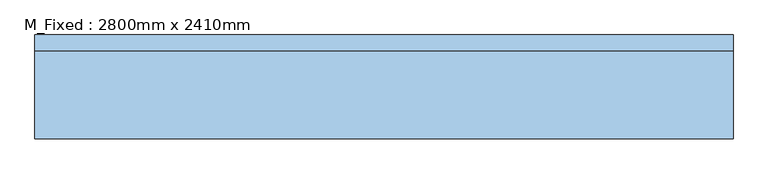
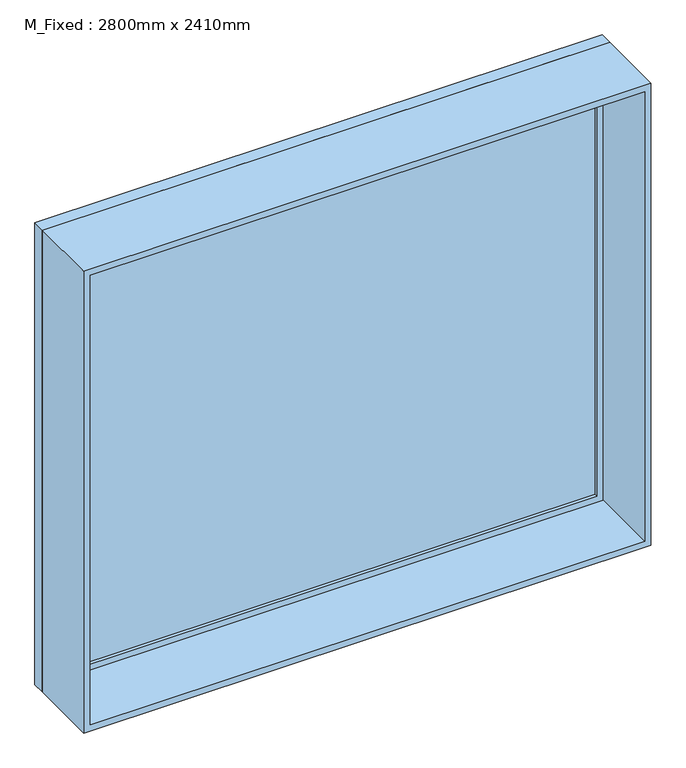
"""IFC4 building model written with IfcOpenShell, lengths in millimetres: window geometry, M_Fixed : 2800mm x 2410mm."""

from ifc_helpers import new_model, si_unit, frame, origin, place, context, project, spatial, polyline, outline, extrude, source, transform, mapped, element, save


def m_fixed_2800mm_x_2410mm_0fa4d817(model_context):
    return source(origin(), model_context, "Body", "SweptSolid", [
        extrude(outline(polyline([(-1337.0, 186.5), (1337.0, 186.5), (1337.0, 174.5), (-1337.0, 174.5), (-1337.0, 186.5)])), frame((0.0, 0.0, 163.0), z_axis=(0.0, 0.0, 1.0), x_axis=(1.0, 0.0, 0.0)), (0.0, 0.0, 1.0), 2284.0),
        extrude(outline(polyline([(2491.0, -1381.0), (119.0, -1381.0), (119.0, 1381.0), (2491.0, 1381.0), (2491.0, -1381.0)]), holes=[polyline([(2447.0, -1337.0), (2447.0, 1337.0), (163.0, 1337.0), (163.0, -1337.0), (2447.0, -1337.0)])]), frame((0.0, 158.5, 0.0), z_axis=(0.0, 1.0, 0.0), x_axis=(0.0, 0.0, 1.0)), (0.0, 0.0, 1.0), 44.0),
        extrude(outline(polyline([(2510.0, -1400.0), (100.0, -1400.0), (100.0, 1400.0), (2510.0, 1400.0), (2510.0, -1400.0)]), holes=[polyline([(2491.0, -1381.0), (2491.0, 1381.0), (119.0, 1381.0), (119.0, -1381.0), (2491.0, -1381.0)])]), frame((0.0, 158.5, 0.0), z_axis=(0.0, 1.0, 0.0), x_axis=(0.0, 0.0, 1.0)), (0.0, 0.0, 1.0), 63.0),
        extrude(outline(polyline([(2510.0, -1400.0), (100.0, -1400.0), (100.0, 1400.0), (2510.0, 1400.0), (2510.0, -1400.0)]), holes=[polyline([(2478.0, -1368.0), (2478.0, 1368.0), (132.0, 1368.0), (132.0, -1368.0), (2478.0, -1368.0)])]), frame((0.0, -195.5, 0.0), z_axis=(0.0, 1.0, 0.0), x_axis=(0.0, 0.0, 1.0)), (0.0, 0.0, 1.0), 354.0),
    ])


if __name__ == "__main__":
    model = new_model("IFC4")
    model_context = context("Model", 3, world=origin())
    ifc_project = project(units=[si_unit("LENGTHUNIT", "METRE", prefix="MILLI")], contexts=[model_context])
    site = spatial("IfcSite", under=ifc_project)
    building = spatial("IfcBuilding", under=site)
    placement = place(None, origin())
    m_fixed_2800mm_x_2410mm_shape = m_fixed_2800mm_x_2410mm_0fa4d817(model_context)
    element("IfcWindow", 1, ObjectType="M_Fixed : 2800mm x 2410mm", at=placement, inside=building, context=model_context, shape_type="MappedRepresentation", body=[
        mapped(m_fixed_2800mm_x_2410mm_shape, transform((0.0, 0.0, 0.0), x_axis=(1.0, 0.0, 0.0), y_axis=(0.0, 1.0, 0.0), z_axis=(0.0, 0.0, 1.0))),
    ])
    save(model, "model.ifc")

# Revit data of these elements
# Type "M_Fixed : 2800mm x 2410mm"
#   Manufacturer = "Manufacturer"
#   Type Mark = "01"
#   Construction Type = "Construction Type"
#   AccessibilityPerformance = "AccessibilityPerformance"
#   CodePerformance = "CodePerformance"
#   ConfigurationType = "ConfigurationType"
#   ConstructionType = "ConstructionType"
#   FireRating = "FireRating"
#   GlazingAreaFraction = "GlazingAreaFraction"
#   OperationType = "OperationType"
#   Area = "Area"
#   Color = "Color"
#   Constituents = "Constituents"
#   Features = "Features"
#   Finish = "Finish"
#   Grade = "Grade"
#   Material = "Material"
#   ModelReference = "ModelReference"
#   NominalHeight = "NominalHeight"
#   NominalLength = "NominalLength"
#   NominalWidth = "NominalWidth"
#   ProductionYear = "ProductionYear"
#   Reference = "Reference"
#   Shape = "Shape"
#   Size = "Size"
#   SustainabilityPerformance = "SustainabilityPerformance"
#   WarrantyDescription = "WarrantyDescription"
#   WarrantyDurationLabor = "WarrantyDurationLabor"
#   WarrantyDurationParts = "WarrantyDurationParts"
#   WarrantyGuarantorLabor = "WarrantyGuarantorLabor"
#   WarrantyGuarantorParts = "WarrantyGuarantorParts"
#   ExpectedLife = "ExpectedLife"
#   ReplacementCost = "ReplacementCost"
#   AssetAccountingType = "FIXED"
#   ModelLabel = "ModelLabel"
#   Height = 2.410 m
#   Default Sill Height = 0.100 m
#   Width = 2.800 m
#   Window Inset = 0.019 m
#   Frame Exterior Material = Sash
#   Frame Interior Material = Sash
#   Glass Pane Material = Glass
#   Sash = Sash
#   Wall Closure = (empty or 0)
# Element 1 (IfcWindow, "M_Fixed : 2800mm x 2410mm")
#   Materials on its faces: "Sash", "Glass"
# Materials
#   "Sash": class "Wood", colour RGB 224 178 126, transparency 0
#   "Glass": class "Glass", colour RGB 0 128 192, transparency 0.9
